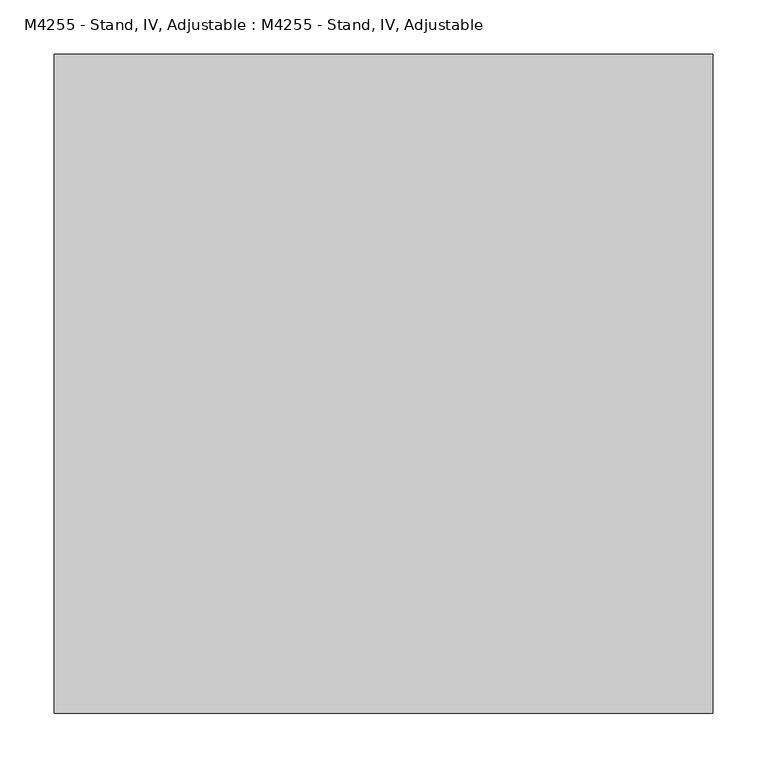
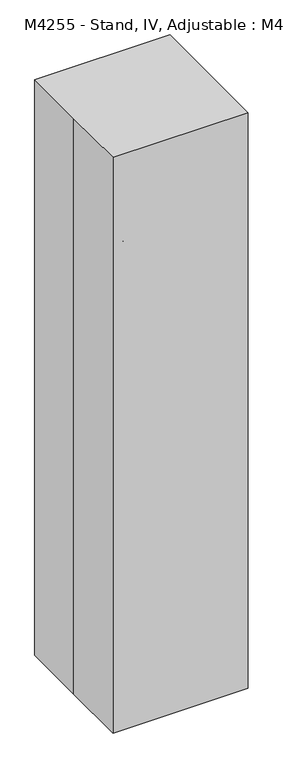
"""IFC4 building model written with IfcOpenShell, lengths in millimetres: proxy geometry, M4255 - Stand, IV, Adjustable : M4255 - Stand, IV, Adjustable."""

from ifc_helpers import new_model, si_unit, point, frame, frame_2d, origin, origin_with_axes, origin_2d, place, context, project, spatial, polyline, circle_curve, ellipse_curve, trimmed, segment, composite_curve, outline, extrude, source, transform, mapped, element, save
from ifc_brep_helpers import plane_surface, cylinder_surface, revolved_surface, advanced_brep


def m4255_stand_iv_adjustable_m4255_stand_iv_adjustable_7ade654a(model_context):
    return source(origin(), model_context, "Body", "SolidModel", [
        extrude(outline(composite_curve([segment(trimmed(circle_curve(frame_2d((25.4, -203.0677083)), 25.4), [point((25.4, -177.6677083))], [point((25.4, -228.4677083))], False, "CARTESIAN"), True, "CONTINUOUS"), segment(trimmed(circle_curve(frame_2d((25.4, -203.0677083)), 25.4), [point((25.4, -228.4677083))], [point((25.4, -177.6677083))], False, "CARTESIAN"), True, "CONTINUOUS")], self_intersect=False)), frame((0.0, -19.05, 0.0), z_axis=(0.0, 1.0, 0.0), x_axis=(0.0, 0.0, 1.0)), (0.0, 0.0, 1.0), 9.525),
        extrude(outline(composite_curve([segment(trimmed(circle_curve(frame_2d((25.4, -203.0677083)), 25.4), [point((25.4, -177.6677083))], [point((25.4, -228.4677083))], False, "CARTESIAN"), True, "CONTINUOUS"), segment(trimmed(circle_curve(frame_2d((25.4, -203.0677083)), 25.4), [point((25.4, -228.4677083))], [point((25.4, -177.6677083))], False, "CARTESIAN"), True, "CONTINUOUS")], self_intersect=False)), frame((0.0, 9.525, 0.0), z_axis=(0.0, 1.0, 0.0), x_axis=(0.0, 0.0, 1.0)), (0.0, 0.0, 1.0), 9.525),
        extrude(outline(composite_curve([segment(trimmed(circle_curve(frame_2d((-203.0677083, 25.4)), 25.4), [point((-228.4677083, 25.4))], [point((-177.6677083, 25.4))], False, "CARTESIAN"), True, "CONTINUOUS"), segment(trimmed(circle_curve(frame_2d((-203.0677083, 25.4)), 25.4), [point((-177.6677083, 25.4))], [point((-228.4677083, 25.4))], False, "CARTESIAN"), True, "CONTINUOUS")], self_intersect=False)), frame((9.525, 0.0, 0.0), z_axis=(1.0, 0.0, 0.0), x_axis=(0.0, 1.0, 0.0)), (0.0, 0.0, 1.0), 9.525),
        extrude(outline(composite_curve([segment(trimmed(circle_curve(frame_2d((-203.0677083, 25.4)), 25.4), [point((-177.6677083, 25.4))], [point((-228.4677083, 25.4))], False, "CARTESIAN"), True, "CONTINUOUS"), segment(trimmed(circle_curve(frame_2d((-203.0677083, 25.4)), 25.4), [point((-228.4677083, 25.4))], [point((-177.6677083, 25.4))], False, "CARTESIAN"), True, "CONTINUOUS")], self_intersect=False)), frame((-19.05, 0.0, 0.0), z_axis=(1.0, 0.0, 0.0), x_axis=(0.0, 1.0, 0.0)), (0.0, 0.0, 1.0), 9.525),
        extrude(outline(composite_curve([segment(trimmed(circle_curve(frame_2d((25.4, 203.2661458)), 25.4), [point((25.4, 228.6661458))], [point((25.4, 177.8661458))], False, "CARTESIAN"), True, "CONTINUOUS"), segment(trimmed(circle_curve(frame_2d((25.4, 203.2661458)), 25.4), [point((25.4, 177.8661458))], [point((25.4, 228.6661458))], False, "CARTESIAN"), True, "CONTINUOUS")], self_intersect=False)), frame((0.0, 9.525, 0.0), z_axis=(0.0, 1.0, 0.0), x_axis=(0.0, 0.0, 1.0)), (0.0, 0.0, 1.0), 9.525),
        extrude(outline(composite_curve([segment(trimmed(circle_curve(frame_2d((25.4, 203.2661458)), 25.4), [point((25.4, 177.8661458))], [point((25.4, 228.6661458))], False, "CARTESIAN"), True, "CONTINUOUS"), segment(trimmed(circle_curve(frame_2d((25.4, 203.2661458)), 25.4), [point((25.4, 228.6661458))], [point((25.4, 177.8661458))], False, "CARTESIAN"), True, "CONTINUOUS")], self_intersect=False)), frame((0.0, -19.05, 0.0), z_axis=(0.0, 1.0, 0.0), x_axis=(0.0, 0.0, 1.0)), (0.0, 0.0, 1.0), 9.525),
        extrude(outline(composite_curve([segment(trimmed(circle_curve(frame_2d((0.0, -211.534375)), 8.4666667), [point((-8.4666667, -211.534375))], [point((8.4666667, -211.534375))], False, "CARTESIAN"), True, "CONTINUOUS"), segment(trimmed(circle_curve(frame_2d((0.0, -211.534375)), 8.4666667), [point((8.4666667, -211.534375))], [point((-8.4666667, -211.534375))], False, "CARTESIAN"), True, "CONTINUOUS")], self_intersect=False)), frame((0.0, 0.0, 25.4), z_axis=(0.0, 0.0, 1.0), x_axis=(1.0, 0.0, 0.0)), (0.0, 0.0, 1.0), 25.4),
        extrude(outline(composite_curve([segment(trimmed(circle_curve(frame_2d((-203.0677083, 25.4)), 16.9333333), [point((-186.134375, 25.4))], [point((-220.0010417, 25.4))], False, "CARTESIAN"), True, "CONTINUOUS"), segment(trimmed(circle_curve(frame_2d((-203.0677083, 25.4)), 16.9333333), [point((-220.0010417, 25.4))], [point((-186.134375, 25.4))], False, "CARTESIAN"), True, "CONTINUOUS")], self_intersect=False)), frame((-9.525, 0.0, 0.0), z_axis=(1.0, 0.0, 0.0), x_axis=(0.0, 1.0, 0.0)), (0.0, 0.0, 1.0), 19.05),
        extrude(outline(composite_curve([segment(trimmed(circle_curve(frame_2d((211.7328125, 0.0)), 8.4666667), [point((211.7328125, -8.4666667))], [point((211.7328125, 8.4666667))], False, "CARTESIAN"), True, "CONTINUOUS"), segment(trimmed(circle_curve(frame_2d((211.7328125, 0.0)), 8.4666667), [point((211.7328125, 8.4666667))], [point((211.7328125, -8.4666667))], False, "CARTESIAN"), True, "CONTINUOUS")], self_intersect=False)), frame((0.0, 0.0, 25.4), z_axis=(0.0, 0.0, 1.0), x_axis=(1.0, 0.0, 0.0)), (0.0, 0.0, 1.0), 25.4),
        extrude(outline(composite_curve([segment(trimmed(circle_curve(frame_2d((25.4, 203.2661458)), 16.9333333), [point((25.4, 186.3328125))], [point((25.4, 220.1994792))], False, "CARTESIAN"), True, "CONTINUOUS"), segment(trimmed(circle_curve(frame_2d((25.4, 203.2661458)), 16.9333333), [point((25.4, 220.1994792))], [point((25.4, 186.3328125))], False, "CARTESIAN"), True, "CONTINUOUS")], self_intersect=False)), frame((0.0, -9.525, 0.0), z_axis=(0.0, 1.0, 0.0), x_axis=(0.0, 0.0, 1.0)), (0.0, 0.0, 1.0), 19.05),
        extrude(outline(composite_curve([segment(trimmed(circle_curve(frame_2d((-211.534375, 0.0)), 8.4666667), [point((-211.534375, 8.4666667))], [point((-211.534375, -8.4666667))], False, "CARTESIAN"), True, "CONTINUOUS"), segment(trimmed(circle_curve(frame_2d((-211.534375, 0.0)), 8.4666667), [point((-211.534375, -8.4666667))], [point((-211.534375, 8.4666667))], False, "CARTESIAN"), True, "CONTINUOUS")], self_intersect=False)), frame((0.0, 0.0, 25.4), z_axis=(0.0, 0.0, 1.0), x_axis=(1.0, 0.0, 0.0)), (0.0, 0.0, 1.0), 25.4),
        extrude(outline(composite_curve([segment(trimmed(circle_curve(frame_2d((25.4, -203.0677083)), 16.9333333), [point((25.4, -186.134375))], [point((25.4, -220.0010417))], False, "CARTESIAN"), True, "CONTINUOUS"), segment(trimmed(circle_curve(frame_2d((25.4, -203.0677083)), 16.9333333), [point((25.4, -220.0010417))], [point((25.4, -186.134375))], False, "CARTESIAN"), True, "CONTINUOUS")], self_intersect=False)), frame((0.0, -9.525, 0.0), z_axis=(0.0, 1.0, 0.0), x_axis=(0.0, 0.0, 1.0)), (0.0, 0.0, 1.0), 19.05),
        extrude(outline(composite_curve([segment(trimmed(circle_curve(frame_2d((203.2165365, 25.4)), 25.4), [point((177.8165365, 25.4))], [point((228.6165365, 25.4))], False, "CARTESIAN"), True, "CONTINUOUS"), segment(trimmed(circle_curve(frame_2d((203.2165365, 25.4)), 25.4), [point((228.6165365, 25.4))], [point((177.8165365, 25.4))], False, "CARTESIAN"), True, "CONTINUOUS")], self_intersect=False)), frame((-19.05, 0.0, 0.0), z_axis=(1.0, 0.0, 0.0), x_axis=(0.0, 1.0, 0.0)), (0.0, 0.0, 1.0), 9.525),
        extrude(outline(composite_curve([segment(trimmed(circle_curve(frame_2d((203.2165365, 25.4)), 25.4), [point((177.8165365, 25.4))], [point((228.6165365, 25.4))], False, "CARTESIAN"), True, "CONTINUOUS"), segment(trimmed(circle_curve(frame_2d((203.2165365, 25.4)), 25.4), [point((228.6165365, 25.4))], [point((177.8165365, 25.4))], False, "CARTESIAN"), True, "CONTINUOUS")], self_intersect=False)), frame((9.525, 0.0, 0.0), z_axis=(1.0, 0.0, 0.0), x_axis=(0.0, 1.0, 0.0)), (0.0, 0.0, 1.0), 9.525),
        extrude(outline(composite_curve([segment(trimmed(circle_curve(frame_2d((0.0, 211.6832031)), 8.4666667), [point((8.4666667, 211.6832031))], [point((-8.4666667, 211.6832031))], False, "CARTESIAN"), True, "CONTINUOUS"), segment(trimmed(circle_curve(frame_2d((0.0, 211.6832031)), 8.4666667), [point((-8.4666667, 211.6832031))], [point((8.4666667, 211.6832031))], False, "CARTESIAN"), True, "CONTINUOUS")], self_intersect=False)), frame((0.0, 0.0, 25.4), z_axis=(0.0, 0.0, 1.0), x_axis=(1.0, 0.0, 0.0)), (0.0, 0.0, 1.0), 25.4),
        extrude(outline(composite_curve([segment(trimmed(circle_curve(frame_2d((203.2165365, 25.4)), 16.9333333), [point((186.2832031, 25.4))], [point((220.1498698, 25.4))], False, "CARTESIAN"), True, "CONTINUOUS"), segment(trimmed(circle_curve(frame_2d((203.2165365, 25.4)), 16.9333333), [point((220.1498698, 25.4))], [point((186.2832031, 25.4))], False, "CARTESIAN"), True, "CONTINUOUS")], self_intersect=False)), frame((-9.525, 0.0, 0.0), z_axis=(1.0, 0.0, 0.0), x_axis=(0.0, 1.0, 0.0)), (0.0, 0.0, 1.0), 19.05),
        extrude(outline(polyline([(228.6, 63.5), (228.6, 50.8), (193.8216772, 50.8), (45.6550105, 12.7), (-45.6550105, 12.7), (-193.8216772, 50.8), (-228.6, 50.8), (-228.6, 63.5), (-192.6166667, 63.5), (-44.45, 25.4), (44.45, 25.4), (192.6166667, 63.5), (228.6, 63.5)])), frame((-19.05, 0.0, 0.0), z_axis=(1.0, 0.0, 0.0), x_axis=(0.0, 1.0, 0.0)), (0.0, 0.0, 1.0), 38.1),
        extrude(outline(composite_curve([segment(trimmed(circle_curve(origin_2d(), 12.7), [point((-12.7, 0.0))], [point((12.7, 0.0))], False, "CARTESIAN"), True, "CONTINUOUS"), segment(trimmed(circle_curve(origin_2d(), 12.7), [point((12.7, 0.0))], [point((-12.7, 0.0))], False, "CARTESIAN"), True, "CONTINUOUS")], self_intersect=False)), frame((0.0, 0.0, 12.7), z_axis=(0.0, 0.0, 1.0), x_axis=(1.0, 0.0, 0.0)), (0.0, 0.0, 1.0), 1473.2),
        extrude(outline(polyline([(63.5, -228.6), (50.8, -228.6), (50.8, -193.8216772), (12.7, -45.6550105), (12.7, 45.6550105), (50.8, 193.8216772), (50.8, 228.6), (63.5, 228.6), (63.5, 192.6166667), (25.4, 44.45), (25.4, -44.45), (63.5, -192.6166667), (63.5, -228.6)])), frame((0.0, -19.05, 0.0), z_axis=(0.0, 1.0, 0.0), x_axis=(0.0, 0.0, 1.0)), (0.0, 0.0, 1.0), 38.1),
        extrude(outline(composite_curve([segment(trimmed(circle_curve(origin_2d(), 6.35), [point((-6.35, 0.0))], [point((6.35, 0.0))], False, "CARTESIAN"), True, "CONTINUOUS"), segment(trimmed(circle_curve(origin_2d(), 6.35), [point((6.35, 0.0))], [point((-6.35, 0.0))], False, "CARTESIAN"), True, "CONTINUOUS")], self_intersect=False)), frame((0.0, 0.0, 1485.9), z_axis=(0.0, 0.0, 1.0), x_axis=(1.0, 0.0, 0.0)), (0.0, 0.0, 1.0), 495.3),
        advanced_brep(
        [(0.0, -117.4754217, 1962.0563468), (0.0, -111.8996536, 1954.3338837), (0.0, -129.4777585, 1941.6421511), (0.0, -135.0535266, 1949.3646141), (0.0, -139.7, 1973.2625), (0.0, -139.7, 1963.7375), (0.0, 139.7, 1973.2625), (0.0, 139.7, 1963.7375), (0.0, 129.4777585, 1941.6421511), (0.0, 135.0535266, 1949.3646141), (0.0, 117.4754217, 1962.0563468), (0.0, 111.8996536, 1954.3338837)],
        [
            (0, 1, circle_curve(frame((0.0, -114.6875376, 1958.1951153), z_axis=(0.0, 0.8107572744902805, 0.5853824748496423), x_axis=(0.0, 0.5853824748496423, -0.8107572744902805)), 4.7625)),
            (1, 0, circle_curve(frame((0.0, -114.6875376, 1958.1951153), z_axis=(0.0, 0.8107572744902805, 0.5853824748496423), x_axis=(0.0, 0.5853824748496423, -0.8107572744902805)), 4.7625)),
            (1, 2),
            (2, 3, circle_curve(frame((0.0, -132.2656426, 1945.5033826), z_axis=(0.0, 0.8107572744902805, 0.5853824748496423), x_axis=(0.0, 0.5853824748496423, -0.8107572744902805)), 4.7625)),
            (3, 0),
            (3, 2, circle_curve(frame((0.0, -132.2656426, 1945.5033826), z_axis=(0.0, 0.8107572744902805, 0.5853824748496423), x_axis=(0.0, 0.5853824748496423, -0.8107572744902805)), 4.7625)),
            (4, 5, circle_curve(frame((0.0, -139.7, 1968.5), z_axis=(0.0, -1.0, 0.0), x_axis=(0.0, 0.0, 1.0)), 4.7625)),
            (5, 3, circle_curve(frame((0.0, -139.7, 1955.8), z_axis=(1.0, 0.0, 0.0), x_axis=(0.0, 0.5853824748496388, -0.810757274490283)), 7.9375)),
            (2, 4, circle_curve(frame((0.0, -139.7, 1955.8), z_axis=(-1.0, 0.0, 0.0), x_axis=(0.0, 0.5853824748496388, -0.810757274490283)), 17.4625)),
            (5, 4, circle_curve(frame((0.0, -139.7, 1968.5), z_axis=(0.0, -1.0, 0.0), x_axis=(0.0, 0.0, 1.0)), 4.7625)),
            (4, 6),
            (6, 7, circle_curve(frame((0.0, 139.7, 1968.5), z_axis=(0.0, -1.0, 0.0), x_axis=(0.0, 0.0, 1.0)), 4.7625)),
            (7, 5),
            (7, 6, circle_curve(frame((0.0, 139.7, 1968.5), z_axis=(0.0, -1.0, 0.0), x_axis=(0.0, 0.0, 1.0)), 4.7625)),
            (8, 9, circle_curve(frame((0.0, 132.2656426, 1945.5033826), z_axis=(0.0, 0.8107572744895747, -0.5853824748506197), x_axis=(0.0, -0.5853824748506197, -0.8107572744895747)), 4.7625)),
            (9, 7, circle_curve(frame((0.0, 139.7, 1955.8), z_axis=(1.0, 0.0, 0.0), x_axis=(0.0, 0.0, 1.0)), 7.9375)),
            (6, 8, circle_curve(frame((0.0, 139.7, 1955.8), z_axis=(-1.0, 0.0, 0.0), x_axis=(0.0, 0.0, 1.0)), 17.4625)),
            (9, 8, circle_curve(frame((0.0, 132.2656426, 1945.5033826), z_axis=(0.0, 0.8107572744906172, -0.5853824748491758), x_axis=(0.0, -0.5853824748491758, -0.8107572744906172)), 4.7625)),
            (10, 11, circle_curve(frame((0.0, 114.6875376, 1958.1951153), z_axis=(0.0, -0.8107572744898955, 0.5853824748501754), x_axis=(0.0, -0.5853824748501754, -0.8107572744898955)), 4.7625)),
            (11, 10, circle_curve(frame((0.0, 114.6875376, 1958.1951153), z_axis=(0.0, -0.8107572744898955, 0.5853824748501754), x_axis=(0.0, -0.5853824748501754, -0.8107572744898955)), 4.7625)),
            (8, 11),
            (10, 9),
        ],
        [
            plane_surface(frame((266.7, -114.6875376, 1958.1951153), z_axis=(0.0, 0.8107572744902805, 0.5853824748496423), x_axis=(-1.0, 0.0, 0.0))),
            cylinder_surface(frame((0.0, -114.6875376, 1958.1951153), z_axis=(0.0, 0.8107572744902805, 0.5853824748496423), x_axis=(0.0, 0.5853824748496423, -0.8107572744902805)), 4.7625),
            revolved_surface(trimmed(ellipse_curve(frame((0.0, -132.2656426, 1945.5033826), z_axis=(0.0, -0.810757274490283, -0.5853824748496388), x_axis=(0.0, 0.5853824748496388, -0.810757274490283)), 4.7625, 4.7625), [point((0.0, -135.0535266, 1949.3646141))], [point((0.0, -129.4777585, 1941.6421511))], True, "CARTESIAN"), (266.7, -139.7, 1955.8), (1.0, 0.0, 0.0)),
            revolved_surface(trimmed(ellipse_curve(frame((0.0, -132.2656426, 1945.5033826), z_axis=(0.0, -0.810757274490283, -0.5853824748496388), x_axis=(0.0, 0.5853824748496388, -0.810757274490283)), 4.7625, 4.7625), [point((0.0, -129.4777585, 1941.6421511))], [point((0.0, -135.0535266, 1949.3646141))], True, "CARTESIAN"), (266.7, -139.7, 1955.8), (1.0, 0.0, 0.0)),
            cylinder_surface(frame((0.0, -139.7, 1968.5), z_axis=(0.0, -1.0, 0.0), x_axis=(0.0, 0.0, 1.0)), 4.7625),
            revolved_surface(trimmed(ellipse_curve(frame((0.0, 139.7, 1968.5), z_axis=(0.0, 1.0, 0.0), x_axis=(0.0, 0.0, 1.0)), 4.7625, 4.7625), [point((0.0, 139.7, 1963.7375))], [point((0.0, 139.7, 1973.2625))], True, "CARTESIAN"), (266.7, 139.7, 1955.8), (1.0, 0.0, 0.0)),
            revolved_surface(trimmed(ellipse_curve(frame((0.0, 139.7, 1968.5), z_axis=(0.0, 1.0, 0.0), x_axis=(0.0, 0.0, 1.0)), 4.7625, 4.7625), [point((0.0, 139.7, 1973.2625))], [point((0.0, 139.7, 1963.7375))], True, "CARTESIAN"), (266.7, 139.7, 1955.8), (1.0, 0.0, 0.0)),
            plane_surface(frame((266.7, 114.6875376, 1958.1951153), z_axis=(0.0, -0.8107572744898955, 0.5853824748501754), x_axis=(-1.0, 0.0, 0.0))),
            cylinder_surface(frame((0.0, 132.2656426, 1945.5033826), z_axis=(0.0, 0.8107572744898955, -0.5853824748501754), x_axis=(0.0, -0.5853824748501754, -0.8107572744898955)), 4.7625),
        ],
        [
            (0, [[1, 2]]),
            (1, [[3, 4, 5, -2]]),
            (1, [[-5, 6, -3, -1]]),
            (2, [[7, 8, -4, 9]]),
            (3, [[10, -9, -6, -8]]),
            (4, [[11, 12, 13, -7]]),
            (4, [[-13, 14, -11, -10]]),
            (5, [[15, 16, -12, 17]]),
            (6, [[18, -17, -14, -16]]),
            (7, [[19, 20]]),
            (8, [[21, -19, 22, -15]]),
            (8, [[-22, -20, -21, -18]]),
        ],
    ),
        advanced_brep(
        [(-117.4754217, 0.0, 1962.0563468), (-111.8996536, 0.0, 1954.3338837), (-129.4777585, 0.0, 1941.6421511), (-135.0535266, 0.0, 1949.3646141), (-139.7, 0.0, 1973.2625), (-139.7, 0.0, 1963.7375), (139.7, 0.0, 1973.2625), (139.7, 0.0, 1963.7375), (129.4777585, 0.0, 1941.6421511), (135.0535266, 0.0, 1949.3646141), (117.4754217, 0.0, 1962.0563468), (111.8996536, 0.0, 1954.3338837)],
        [
            (0, 1, circle_curve(frame((-114.6875376, 0.0, 1958.1951153), z_axis=(0.810757274490287, 0.0, 0.5853824748496333), x_axis=(0.5853824748496333, 0.0, -0.810757274490287)), 4.7625)),
            (1, 0, circle_curve(frame((-114.6875376, 0.0, 1958.1951153), z_axis=(0.810757274490287, 0.0, 0.5853824748496333), x_axis=(0.5853824748496333, 0.0, -0.810757274490287)), 4.7625)),
            (1, 2),
            (2, 3, circle_curve(frame((-132.2656426, 0.0, 1945.5033826), z_axis=(0.810757274490287, 0.0, 0.5853824748496333), x_axis=(0.5853824748496333, 0.0, -0.810757274490287)), 4.7625)),
            (3, 0),
            (3, 2, circle_curve(frame((-132.2656426, 0.0, 1945.5033826), z_axis=(0.810757274490287, 0.0, 0.5853824748496333), x_axis=(0.5853824748496333, 0.0, -0.810757274490287)), 4.7625)),
            (4, 5, circle_curve(frame((-139.7, 0.0, 1968.5), z_axis=(-1.0, 0.0, 0.0), x_axis=(0.0, 0.0, 1.0)), 4.7625)),
            (5, 3, circle_curve(frame((-139.7, 0.0, 1955.8), z_axis=(0.0, -1.0, 0.0), x_axis=(0.5853824748496308, 0.0, -0.8107572744902887)), 7.9375)),
            (2, 4, circle_curve(frame((-139.7, 0.0, 1955.8), z_axis=(0.0, 1.0, 0.0), x_axis=(0.5853824748496308, 0.0, -0.8107572744902887)), 17.4625)),
            (5, 4, circle_curve(frame((-139.7, 0.0, 1968.5), z_axis=(-1.0, 0.0, 0.0), x_axis=(0.0, 0.0, 1.0)), 4.7625)),
            (4, 6),
            (6, 7, circle_curve(frame((139.7, 0.0, 1968.5), z_axis=(-1.0, 0.0, 0.0), x_axis=(0.0, 0.0, 1.0)), 4.7625)),
            (7, 5),
            (7, 6, circle_curve(frame((139.7, 0.0, 1968.5), z_axis=(-1.0, 0.0, 0.0), x_axis=(0.0, 0.0, 1.0)), 4.7625)),
            (8, 9, circle_curve(frame((132.2656426, 0.0, 1945.5033826), z_axis=(0.8107572744899039, 0.0, -0.5853824748501637), x_axis=(-0.5853824748501637, 0.0, -0.8107572744899039)), 4.7625)),
            (9, 7, circle_curve(frame((139.7, 0.0, 1955.8), z_axis=(0.0, -1.0, 0.0), x_axis=(0.0, 0.0, 1.0)), 7.9375)),
            (6, 8, circle_curve(frame((139.7, 0.0, 1955.8), z_axis=(0.0, 1.0, 0.0), x_axis=(0.0, 0.0, 1.0)), 17.4625)),
            (9, 8, circle_curve(frame((132.2656426, 0.0, 1945.5033826), z_axis=(0.8107572744899008, 0.0, -0.585382474850168), x_axis=(-0.585382474850168, 0.0, -0.8107572744899008)), 4.7625)),
            (10, 11, circle_curve(frame((114.6875376, 0.0, 1958.1951153), z_axis=(-0.8107572744899005, 0.0, 0.5853824748501685), x_axis=(-0.5853824748501685, 0.0, -0.8107572744899005)), 4.7625)),
            (11, 10, circle_curve(frame((114.6875376, 0.0, 1958.1951153), z_axis=(-0.8107572744899005, 0.0, 0.5853824748501685), x_axis=(-0.5853824748501685, 0.0, -0.8107572744899005)), 4.7625)),
            (8, 11),
            (10, 9),
        ],
        [
            plane_surface(frame((-114.6875376, -215.9, 1958.1951153), z_axis=(0.810757274490287, 0.0, 0.5853824748496333), x_axis=(0.0, 1.0, 0.0))),
            cylinder_surface(frame((-114.6875376, 0.0, 1958.1951153), z_axis=(0.810757274490287, 0.0, 0.5853824748496333), x_axis=(0.5853824748496333, 0.0, -0.810757274490287)), 4.7625),
            revolved_surface(trimmed(ellipse_curve(frame((-132.2656426, 0.0, 1945.5033826), z_axis=(-0.8107572744902886, 0.0, -0.585382474849631), x_axis=(0.585382474849631, 0.0, -0.8107572744902886)), 4.7625, 4.7625), [point((-135.0535266, 0.0, 1949.3646141))], [point((-129.4777585, 0.0, 1941.6421511))], True, "CARTESIAN"), (-139.7, -215.9, 1955.8), (0.0, -1.0, 0.0)),
            revolved_surface(trimmed(ellipse_curve(frame((-132.2656426, 0.0, 1945.5033826), z_axis=(-0.8107572744902886, 0.0, -0.585382474849631), x_axis=(0.585382474849631, 0.0, -0.8107572744902886)), 4.7625, 4.7625), [point((-129.4777585, 0.0, 1941.6421511))], [point((-135.0535266, 0.0, 1949.3646141))], True, "CARTESIAN"), (-139.7, -215.9, 1955.8), (0.0, -1.0, 0.0)),
            cylinder_surface(frame((-139.7, 0.0, 1968.5), z_axis=(-1.0, 0.0, 0.0), x_axis=(0.0, 0.0, 1.0)), 4.7625),
            revolved_surface(trimmed(ellipse_curve(frame((139.7, 0.0, 1968.5), z_axis=(1.0, 0.0, 0.0), x_axis=(0.0, 0.0, 1.0)), 4.7625, 4.7625), [point((139.7, 0.0, 1963.7375))], [point((139.7, 0.0, 1973.2625))], True, "CARTESIAN"), (139.7, -215.9, 1955.8), (0.0, -1.0, 0.0)),
            revolved_surface(trimmed(ellipse_curve(frame((139.7, 0.0, 1968.5), z_axis=(1.0, 0.0, 0.0), x_axis=(0.0, 0.0, 1.0)), 4.7625, 4.7625), [point((139.7, 0.0, 1973.2625))], [point((139.7, 0.0, 1963.7375))], True, "CARTESIAN"), (139.7, -215.9, 1955.8), (0.0, -1.0, 0.0)),
            plane_surface(frame((114.6875376, -215.9, 1958.1951153), z_axis=(-0.8107572744899004, 0.0, 0.5853824748501686), x_axis=(0.0, 1.0, 0.0))),
            cylinder_surface(frame((132.2656426, 0.0, 1945.5033826), z_axis=(0.8107572744899005, 0.0, -0.5853824748501685), x_axis=(-0.5853824748501685, 0.0, -0.8107572744899005)), 4.7625),
        ],
        [
            (0, [[1, 2]]),
            (1, [[3, 4, 5, -2]]),
            (1, [[-5, 6, -3, -1]]),
            (2, [[7, 8, -4, 9]]),
            (3, [[10, -9, -6, -8]]),
            (4, [[11, 12, 13, -7]]),
            (4, [[-13, 14, -11, -10]]),
            (5, [[15, 16, -12, 17]]),
            (6, [[18, -17, -14, -16]]),
            (7, [[19, 20]]),
            (8, [[21, -19, 22, -15]]),
            (8, [[-22, -20, -21, -18]]),
        ],
    ),
        extrude(outline(polyline([(-304.8, -304.8), (-304.8, 0.0), (-304.8, 304.8), (304.8, 304.8), (304.8, -304.8), (-304.8, -304.8)])), origin_with_axes(), (0.0, 0.0, 1.0), 2743.2),
    ])


if __name__ == "__main__":
    model = new_model("IFC4")
    model_context = context("Model", 3, world=origin())
    ifc_project = project(units=[si_unit("LENGTHUNIT", "METRE", prefix="MILLI")], contexts=[model_context])
    site = spatial("IfcSite", under=ifc_project)
    building = spatial("IfcBuilding", under=site)
    placement = place(None, origin())
    m4255_stand_iv_adjustable_m4255_stand_iv_adjustable_shape = m4255_stand_iv_adjustable_m4255_stand_iv_adjustable_7ade654a(model_context)
    element("IfcBuildingElementProxy", 1, Name="M4255 - Stand, IV, Adjustable : M4255 - Stand, IV, Adjustable", ObjectType="M4255 - Stand, IV, Adjustable : M4255 - Stand, IV, Adjustable", at=placement, inside=building, context=model_context, shape_type="MappedRepresentation", body=[
        mapped(m4255_stand_iv_adjustable_m4255_stand_iv_adjustable_shape, transform((0.0, 0.0, 0.0), x_axis=(1.0, 0.0, 0.0), y_axis=(0.0, 1.0, 0.0), z_axis=(0.0, 0.0, 1.0))),
    ])
    save(model, "model.ifc")

# Revit data of these elements
# Type "M4255 - Stand, IV, Adjustable : M4255 - Stand, IV, Adjustable"
#   Watts2 = "0"
#   Watts1 = "0"
#   Unit_Issue = "EA"
#   UTIL_6_Misc = "-"
#   UTIL_5_NonMedGas = "-"
#   UTIL_4_MiscGas = "-"
#   UTIL_3_MedGas = "-"
#   UTIL_2_Elec = "-"
#   UTIL_1_WaterDrain = "-"
#   Nomenclature = "Stand, IV, Adjustable"
#   NSN = "6530"
#   Location [instance default] = ""
#   JSN = "M4255"
#   Fund_Source_VA = "-"
#   Fund_Source_Navy = "-"
#   Fund_Source_Army = "-"
#   Fund_Source_AF = "-"
#   ELEC_Volts2 = "0"
#   ELEC_Volts1 = "0"
#   ELEC_Phase2 = "0"
#   ELEC_Phase1 = "0"
#   ELEC_HertzSwitch = "0"
#   ELEC_HertzDependent = "0"
#   ELEC_Hertz = "0"
#   ELEC_Amps2 = "0"
#   ELEC_Amps1 = "0"
#   DetailDescription = "Adjustable IV stand with 4-hook arrangement. Stand has stainless steel construction with heavy weight base. It adjusts from 66 inches to 100 inches and is mounted on conductive rubber, ball bearing, swivel casters. Stand is used for administering intravenous solutions."
#   CAT_VA = "C"
#   CAT_Navy = "C"
#   CAT_IHS = "-"
#   CAT_Army = "C"
#   CAT_AF = "C"
#   BTUperhour = "0"
#   radius = 0' - 1"
#   calc 2 = 0' - 0.33333"
#   calc 1 = 0' - 0.66667"
#   Weight_IP = 35
#   DIM_Width_IP = 2' - 0"
#   DIM_Height_IP = 9' - 0"
#   DIM_Depth_IP = 2' - 0"
#   finish [instance default] = none
# Element 1 (IfcBuildingElementProxy, "M4255 - Stand, IV, Adjustable : M4255 - Stand, IV, Adjustable")
#   Location = "BRII2"
#   Materials on its faces: "EquipSpace"
# Materials
#   "EquipSpace": class "Unassigned", colour RGB 221 217 195, transparency 0.5
